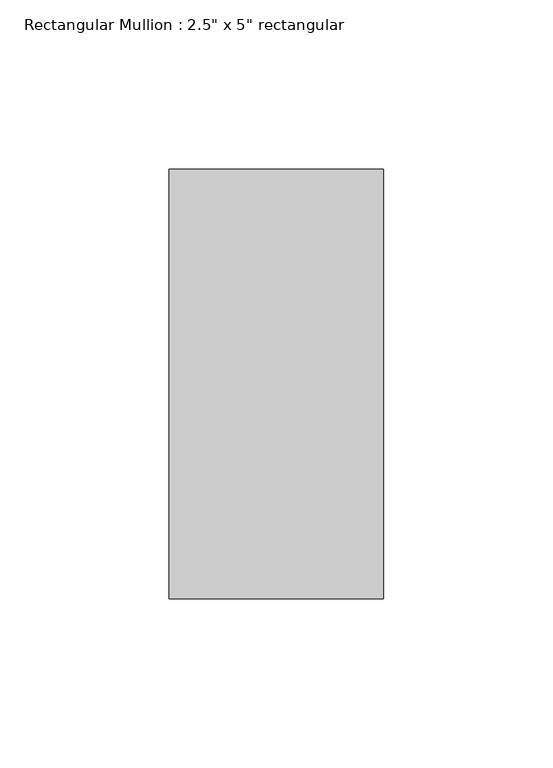
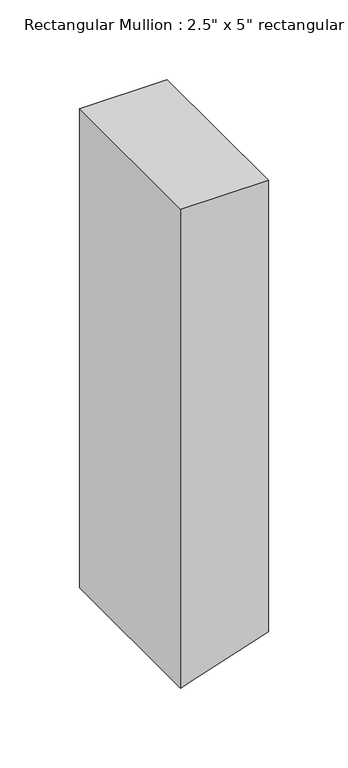
"""IFC4 building model written with IfcOpenShell, lengths in millimetres: member geometry."""

from ifc_helpers import new_model, si_unit, frame, origin, place, context, project, spatial, polyline, outline, extrude, source, transform, mapped, element, save


def member_4067c595(model_context):
    return source(origin(), model_context, "Body", "SweptSolid", [
        extrude(outline(polyline([(0.0, 31.75), (0.0, -31.75), (-366.9817895, -31.75), (-363.0919439, -20.0804631), (-345.8151229, 31.75), (0.0, 31.75)])), frame((0.0, -63.5, 0.0), z_axis=(0.0, 1.0, 0.0), x_axis=(0.0, 0.0, 1.0)), (0.0, 0.0, 1.0), 127.0),
    ])


if __name__ == "__main__":
    model = new_model("IFC4")
    model_context = context("Model", 3, world=origin())
    ifc_project = project(units=[si_unit("LENGTHUNIT", "METRE", prefix="MILLI")], contexts=[model_context])
    site = spatial("IfcSite", under=ifc_project)
    building = spatial("IfcBuilding", under=site)
    placement = place(None, origin())
    member_shape = member_4067c595(model_context)
    element("IfcMember", 1, ObjectType="Rectangular Mullion : 2.5\" x 5\" rectangular", at=placement, inside=building, context=model_context, shape_type="MappedRepresentation", body=[
        mapped(member_shape, transform((0.0, 0.0, 0.0), x_axis=(1.0, 0.0, 0.0), y_axis=(0.0, 1.0, 0.0), z_axis=(0.0, 0.0, 1.0))),
    ])
    save(model, "model.ifc")

# Revit data of these elements
# Type "Rectangular Mullion : 2.5\" x 5\" rectangular"
#   built-in parameter 1007304 = 0.416667 (stored number, unit not read)
#   built-in parameter 1007301 = 0.104167 (stored number, unit not read)
#   built-in parameter 1007300 = 0.104167 (stored number, unit not read)
# Element 1 (IfcMember, "Rectangular Mullion : 2.5\" x 5\" rectangular")
#   Materials on its faces: "Metal - Aluminum"
# Materials
#   "Metal - Aluminum": class "Metal", colour RGB 140 140 140, transparency 0
